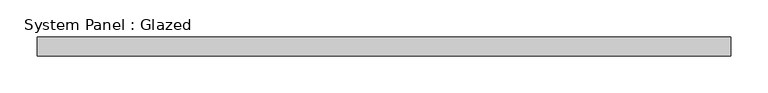
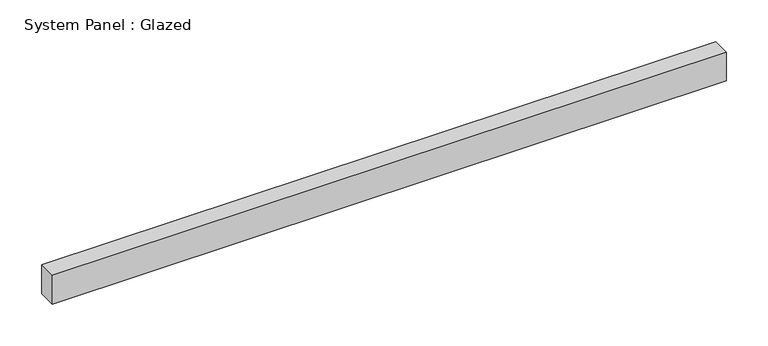
"""IFC4 building model written with IfcOpenShell, lengths in millimetres: plate geometry, System Panel : Glazed."""

from ifc_helpers import new_model, si_unit, origin, origin_with_axes, place, context, project, spatial, polyline, outline, extrude, source, transform, mapped, element, save


def system_panel_glazed_c48c36d0(model_context):
    return source(origin(), model_context, "Body", "SweptSolid", [
        extrude(outline(polyline([(465.8483058, -44.45), (-465.8483058, -44.45), (-465.8483058, -19.05), (465.8483058, -19.05), (465.8483058, -44.45)])), origin_with_axes(), (0.0, 0.0, 1.0), 41.9143134),
    ])


if __name__ == "__main__":
    model = new_model("IFC4")
    model_context = context("Model", 3, world=origin())
    ifc_project = project(units=[si_unit("LENGTHUNIT", "METRE", prefix="MILLI")], contexts=[model_context])
    site = spatial("IfcSite", under=ifc_project)
    building = spatial("IfcBuilding", under=site)
    placement = place(None, origin())
    system_panel_glazed_shape = system_panel_glazed_c48c36d0(model_context)
    element("IfcPlate", 1, ObjectType="System Panel : Glazed", at=placement, inside=building, context=model_context, shape_type="MappedRepresentation", body=[
        mapped(system_panel_glazed_shape, transform((0.0, 0.0, 0.0), x_axis=(1.0, 0.0, 0.0), y_axis=(0.0, 1.0, 0.0), z_axis=(0.0, 0.0, 1.0))),
    ])
    save(model, "model.ifc")

# Revit data of these elements
# Type "System Panel : Glazed"
#   Construction Type Id = "GSP4R"
#   Analytic Construction = "1/8 in Pilkington single glazing"
#   Visual Light Transmittance = 0.9
#   Solar Heat Gain Coefficient = 0.86
#   Heat Transfer Coefficient (U) = 1.18115 BTU/(h·ft²·°F)
#   Define Thermal Properties by = 1
# Element 1 (IfcPlate, "System Panel : Glazed")
#   Materials on its faces: "Glass"
# Materials
#   "Glass": class "Glass", colour RGB 0 128 192, transparency 0.75, Description = "Soda Lime Glass", Cost = 0
